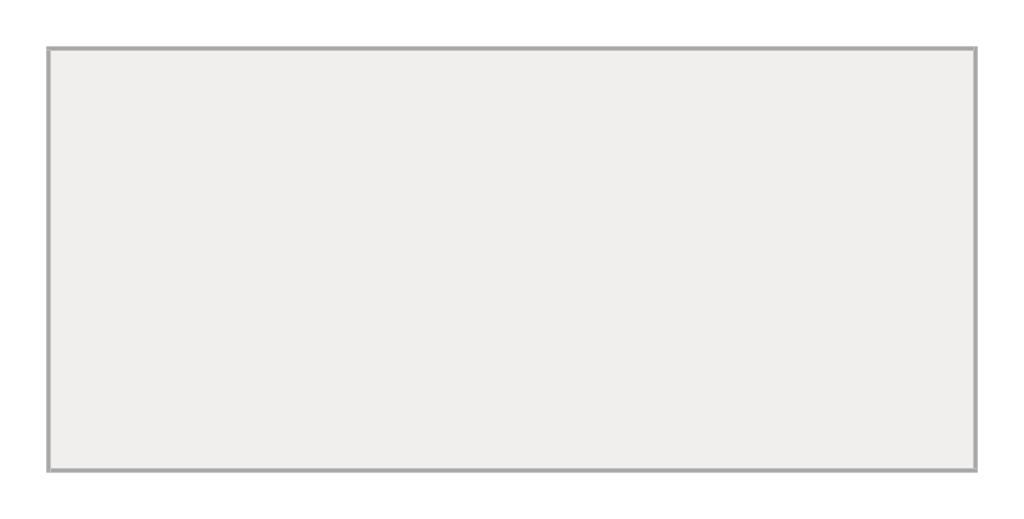
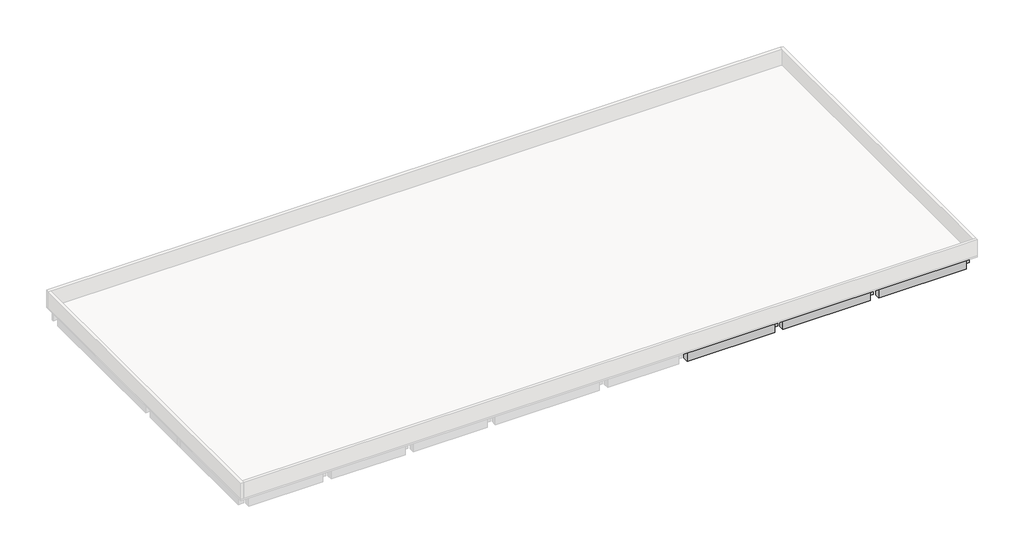
# One storey, part 2 of 2: 30 beams.
"""IFC4 building model written with IfcOpenShell, lengths in millimetres."""

import ifcopenshell
import ifcopenshell.guid

model = None  # the IFC model being written
_history = None  # IfcOwnerHistory: only IFC2X3 demands one
_inside = {}  # id of a spatial element -> (the spatial element, [elements in it])
_under = {}  # id of a project, library or spatial element -> (it, [spatial elements below it])
_declared = {}  # id of a project -> (the project, [libraries it declares])
_typed = {}  # id of a type object -> (the type object, [elements of that type])
_made_of = {}  # id of a material, layer set ... -> (it, [elements and type objects made of it])


def new_model(schema):
    """Start an empty IFC model of exactly this schema.

    Asked for "IFC4X3", IfcOpenShell would pick the latest addendum, in which some entities
    have other attributes; the version numbers below select the first issue.
    IFC2X3 requires an IfcOwnerHistory on every rooted entity: one is made here for all.
    """
    global model, _history
    if schema == "IFC4X3":
        model = ifcopenshell.file(schema_version=(4, 3, 0, 0))
    else:
        model = ifcopenshell.file(schema=schema)
    _inside.clear()
    _under.clear()
    _declared.clear()
    _typed.clear()
    _made_of.clear()
    _history = None
    if model.schema == "IFC2X3":
        org = make("IfcOrganization", Name="unknown")
        user = make(
            "IfcPersonAndOrganization",
            ThePerson=make("IfcPerson", FamilyName="unknown"),
            TheOrganization=org,
        )
        app = make(
            "IfcApplication",
            ApplicationDeveloper=org,
            Version="unknown",
            ApplicationFullName="unknown",
            ApplicationIdentifier="unknown",
        )
        _history = make(
            "IfcOwnerHistory",
            OwningUser=user,
            OwningApplication=app,
            ChangeAction="ADDED",
            CreationDate=0,
        )
    return model


def make(cls, **values):
    """One entity of the class cls with the attributes given. An attribute that is None is left unset."""
    return model.create_entity(
        cls, **{name: value for name, value in values.items() if value is not None}
    )


def rooted(cls, **values):
    """An entity with a GlobalId (a new one), such as an element, a storey or a relation."""
    return make(cls, GlobalId=ifcopenshell.guid.new(), OwnerHistory=_history, **values)


def si_unit(unit_type, name, prefix=None):
    """IfcSIUnit, for example si_unit("LENGTHUNIT", "METRE", prefix="MILLI")."""
    return make("IfcSIUnit", UnitType=unit_type, Prefix=prefix, Name=name)


def assignment(units):
    """IfcUnitAssignment: the units of a project."""
    return None if units is None else make("IfcUnitAssignment", Units=units)


def point(xyz):
    """IfcCartesianPoint."""
    return None if xyz is None else make("IfcCartesianPoint", Coordinates=xyz)


def direction(xyz):
    """IfcDirection."""
    return None if xyz is None else make("IfcDirection", DirectionRatios=xyz)


def frame(location, z_axis=None, x_axis=None):
    """IfcAxis2Placement3D, a coordinate frame: its origin and axes. An axis left out is left unset."""
    return make(
        "IfcAxis2Placement3D",
        Location=point(location),
        Axis=direction(z_axis),
        RefDirection=direction(x_axis),
    )


def origin():
    """The frame at (0, 0, 0) with its axes left unset."""
    return frame((0.0, 0.0, 0.0))


def place(relative_to, where):
    """IfcLocalPlacement: puts the frame where relative to a parent placement (None: the world)."""
    return make(
        "IfcLocalPlacement", PlacementRelTo=relative_to, RelativePlacement=where
    )


def context(
    kind, dimensions, precision=None, world=None, true_north=None, identifier=None
):
    """IfcGeometricRepresentationContext, for example the 3D "Model" context."""
    return make(
        "IfcGeometricRepresentationContext",
        ContextIdentifier=identifier,
        ContextType=kind,
        CoordinateSpaceDimension=dimensions,
        Precision=precision,
        WorldCoordinateSystem=world,
        TrueNorth=true_north,
    )


def project(units=None, contexts=None):
    """IfcProject with its units and contexts."""
    return rooted(
        "IfcProject",
        Name="project",
        RepresentationContexts=contexts,
        UnitsInContext=assignment(units),
    )


def spatial(cls, under=None, at=None, **own):
    """A site, building, storey or space (cls), placed at a placement, below another one or the project."""
    s = rooted(cls, ObjectPlacement=at, **own)
    if under is not None:
        _under.setdefault(under.id(), (under, []))[1].append(s)
    return s


def polyline(points):
    """IfcPolyline through the points."""
    return make("IfcPolyline", Points=[point(p) for p in points])


def outline(outer, holes=None, kind="AREA"):
    """IfcArbitraryClosedProfileDef: a profile drawn as a closed curve; with holes, ...WithVoids."""
    if holes is None:
        return make("IfcArbitraryClosedProfileDef", ProfileType=kind, OuterCurve=outer)
    return make(
        "IfcArbitraryProfileDefWithVoids",
        ProfileType=kind,
        OuterCurve=outer,
        InnerCurves=holes,
    )


def extrude(swept, where, along, depth):
    """IfcExtrudedAreaSolid: the profile swept, set in the frame where, extruded along a direction by depth."""
    return make(
        "IfcExtrudedAreaSolid",
        SweptArea=swept,
        Position=where,
        ExtrudedDirection=direction(along),
        Depth=depth,
    )


def faces_of(points, faces, orient=None, outer=None):
    """IfcFace entities. A face is a list of loops; a loop is a list of indices into points, from 0.

    orient and outer hold one flag for each loop. By default every Orientation is true, the
    first loop of a face is its IfcFaceOuterBound and the others are IfcFaceBound.
    """
    made = []
    for i, loops in enumerate(faces):
        bounds = []
        for j, loop in enumerate(loops):
            is_outer = j == 0 if outer is None else outer[i][j]
            bounds.append(
                make(
                    "IfcFaceOuterBound" if is_outer else "IfcFaceBound",
                    Bound=make("IfcPolyLoop", Polygon=[points[k] for k in loop]),
                    Orientation=True if orient is None else orient[i][j],
                )
            )
        made.append(make("IfcFace", Bounds=bounds))
    return made


def faceted_brep(points, faces, orient=None, outer=None, voids=None):
    """IfcFacetedBrep: a solid bounded by flat faces; with voids (closed shells), ...WithVoids."""
    shared = [point(p) for p in points]
    hull = make("IfcClosedShell", CfsFaces=faces_of(shared, faces, orient, outer))
    if voids is None:
        return make("IfcFacetedBrep", Outer=hull)
    return make(
        "IfcFacetedBrepWithVoids",
        Outer=hull,
        Voids=[
            make(cls, CfsFaces=faces_of(shared, fs, o, b)) for cls, fs, o, b in voids
        ],
    )


def shape(context_of_items, identifier, shape_type, items):
    """IfcShapeRepresentation: the items that make up one representation, for example the "Body"."""
    return make(
        "IfcShapeRepresentation",
        ContextOfItems=context_of_items,
        RepresentationIdentifier=identifier,
        RepresentationType=shape_type,
        Items=items,
    )


def made_of(thing, what):
    """Note that an element or type object is made of a material, layer set ...; save() writes the relation."""
    if what is not None:
        _made_of.setdefault(what.id(), (what, []))[1].append(thing)
    return thing


def element(
    cls,
    number,
    at=None,
    inside=None,
    cuts=None,
    type_object=None,
    material=None,
    context=None,
    identifier="Body",
    shape_type=None,
    held_by="IfcProductDefinitionShape",
    body=None,
    shapes=None,
    **own,
):
    """One element of the class cls, such as IfcWall. Its Tag is "e" and its number.

    at: its placement. inside: the storey or other place that contains it. cuts: it is an
    opening in that element (IfcRelVoidsElement). A single representation is given by context,
    identifier, shape_type and body (its items); several are given by shapes. held_by: the class
    of the entity that holds the representations. save() writes the other relations.
    """
    e = rooted(cls, Tag="e%d" % number, ObjectPlacement=at, **own)
    if body is not None:
        shapes = [shape(context, identifier, shape_type, body)]
    if shapes is not None:
        e.Representation = make(held_by, Representations=shapes)
    if inside is not None:
        _inside.setdefault(inside.id(), (inside, []))[1].append(e)
    if cuts is not None:
        rooted(
            "IfcRelVoidsElement", RelatingBuildingElement=cuts, RelatedOpeningElement=e
        )
    if type_object is not None:
        _typed.setdefault(type_object.id(), (type_object, []))[1].append(e)
    return made_of(e, material)


def aggregate(whole, parts):
    """IfcRelAggregates: a whole, such as a stair, and the parts it consists of."""
    return rooted("IfcRelAggregates", RelatingObject=whole, RelatedObjects=parts)


def save(model, path):
    """Write the relations noted so far, then the file.

    IfcRelAggregates (storeys below a building ...), IfcRelContainedInSpatialStructure (elements
    in a storey), IfcRelDefinesByType, IfcRelAssociatesMaterial and IfcRelDeclares: one each for
    every whole, place, type object, material and project.
    """
    for whole, parts in _under.values():
        aggregate(whole, parts)
    for where, things in _inside.values():
        rooted(
            "IfcRelContainedInSpatialStructure",
            RelatedElements=things,
            RelatingStructure=where,
        )
    for kind, things in _typed.values():
        rooted("IfcRelDefinesByType", RelatedObjects=things, RelatingType=kind)
    for what, things in _made_of.values():
        rooted("IfcRelAssociatesMaterial", RelatedObjects=things, RelatingMaterial=what)
    for by, libraries in _declared.values():
        rooted("IfcRelDeclares", RelatingContext=by, RelatedDefinitions=libraries)
    model.write(path)


model = new_model("IFC4")

# Units and contexts
model_context = context("Model", 3, world=origin())
ifc_project = project(units=[si_unit("LENGTHUNIT", "METRE", prefix="MILLI")], contexts=[model_context])

# Site, building, storey
site = spatial("IfcSite", under=ifc_project)
building = spatial("IfcBuilding", under=site)
storey = spatial("IfcBuildingStorey", under=building, Name="TOC", Elevation=7650.0)

# Beams
placement = place(None, origin())
element("IfcBeam", 1, ObjectType="RC Beam_Rectangular : H_SB_ACB_B400xH900", at=placement, inside=storey, context=model_context, shape_type="Brep", body=[
    faceted_brep([(39124.7, 12116.5208589, 6750.0), (39124.7, 12116.5208589, 7549.0), (38724.7, 12116.5208589, 7549.0), (32124.7, 12116.5208589, 7549.0), (32124.7, 12116.5208589, 6750.0), (38724.7, 12116.5208589, 6750.0), (39124.7, 12516.5208589, 6750.0), (32124.7, 12516.5208589, 6750.0), (38724.7, 12516.5208589, 6750.0), (39124.7, 12516.5208589, 7549.0), (32124.7, 12516.5208589, 7549.0), (38724.7, 12516.5208589, 7549.0)], [[[0, 1, 2, 3, 4, 5]], [[6, 0, 5, 4, 7, 8]], [[9, 6, 8, 7, 10, 11]], [[1, 9, 11, 10, 3, 2]], [[0, 6, 9, 1]], [[4, 3, 10, 7]]]),
])
element("IfcBeam", 2, ObjectType="RC Beam_Rectangular : H_SB_ACB_B400xH900", at=placement, inside=storey, context=model_context, shape_type="Brep", body=[
    faceted_brep([(46124.7, 12116.5208589, 6750.0), (46124.7, 12116.5208589, 7549.0), (45724.7, 12116.5208589, 7549.0), (39124.7, 12116.5208589, 7549.0), (39124.7, 12116.5208589, 6750.0), (45724.7, 12116.5208589, 6750.0), (46124.7, 12516.5208589, 6750.0), (39124.7, 12516.5208589, 6750.0), (45724.7, 12516.5208589, 6750.0), (46124.7, 12516.5208589, 7549.0), (39124.7, 12516.5208589, 7549.0), (45724.7, 12516.5208589, 7549.0)], [[[0, 1, 2, 3, 4, 5]], [[6, 0, 5, 4, 7, 8]], [[9, 6, 8, 7, 10, 11]], [[1, 9, 11, 10, 3, 2]], [[0, 6, 9, 1]], [[4, 3, 10, 7]]]),
])
element("IfcBeam", 3, ObjectType="RC Beam_Rectangular : H_SB_ACB_B400xH900", at=placement, inside=storey, context=model_context, shape_type="Brep", body=[
    faceted_brep([(53124.7, 12116.5208589, 6750.0), (53124.7, 12116.5208589, 7549.0), (52724.7, 12116.5208589, 7549.0), (46124.7, 12116.5208589, 7549.0), (46124.7, 12116.5208589, 6750.0), (52724.7, 12116.5208589, 6750.0), (53124.7, 12516.5208589, 6750.0), (46124.7, 12516.5208589, 6750.0), (52724.7, 12516.5208589, 6750.0), (53124.7, 12516.5208589, 7549.0), (46124.7, 12516.5208589, 7549.0), (52724.7, 12516.5208589, 7549.0)], [[[0, 1, 2, 3, 4, 5]], [[6, 0, 5, 4, 7, 8]], [[9, 6, 8, 7, 10, 11]], [[1, 9, 11, 10, 3, 2]], [[0, 6, 9, 1]], [[4, 3, 10, 7]]]),
])
element("IfcBeam", 4, ObjectType="RC Beam_Rectangular : H_SB_ACB_B400xH900", at=placement, inside=storey, context=model_context, shape_type="SweptSolid", body=[
    extrude(outline(polyline([(7500.0, 224.7), (6750.0, 224.7), (6750.0, 5624.7), (7500.0, 5624.7), (7500.0, 5724.7), (7549.0, 5724.7), (7549.0, 124.7), (7500.0, 124.7), (7500.0, 224.7)])), frame((0.0, 23816.5208589, 0.0), z_axis=(0.0, 1.0, 0.0), x_axis=(0.0, 0.0, 1.0)), (0.0, 0.0, 1.0), 400.0),
])
element("IfcBeam", 5, ObjectType="RC Beam_Rectangular : H_SB_ACB_B400xH900", at=placement, inside=storey, context=model_context, shape_type="SweptSolid", body=[
    extrude(outline(polyline([(7500.0, 6224.7), (6750.0, 6224.7), (6750.0, 11624.7), (7500.0, 11624.7), (7500.0, 11724.7), (7549.0, 11724.7), (7549.0, 6124.7), (7500.0, 6124.7), (7500.0, 6224.7)])), frame((0.0, 23816.5208589, 0.0), z_axis=(0.0, 1.0, 0.0), x_axis=(0.0, 0.0, 1.0)), (0.0, 0.0, 1.0), 400.0),
])
element("IfcBeam", 6, ObjectType="RC Beam_Rectangular : H_SB_ACB_B400xH900", at=placement, inside=storey, context=model_context, shape_type="SweptSolid", body=[
    extrude(outline(polyline([(7500.0, 12224.7), (6750.0, 12224.7), (6750.0, 17624.7), (7500.0, 17624.7), (7500.0, 17724.7), (7549.0, 17724.7), (7549.0, 12124.7), (7500.0, 12124.7), (7500.0, 12224.7)])), frame((0.0, 23816.5208589, 0.0), z_axis=(0.0, 1.0, 0.0), x_axis=(0.0, 0.0, 1.0)), (0.0, 0.0, 1.0), 400.0),
])
element("IfcBeam", 7, ObjectType="RC Beam_Rectangular : H_SB_ACB_B400xH900", at=placement, inside=storey, context=model_context, shape_type="SweptSolid", body=[
    extrude(outline(polyline([(7500.0, 18224.7), (6750.0, 18224.7), (6750.0, 25824.7), (7500.0, 25824.7), (7500.0, 25924.7), (7549.0, 25924.7), (7549.0, 18124.7), (7500.0, 18124.7), (7500.0, 18224.7)])), frame((0.0, 23816.5208589, 0.0), z_axis=(0.0, 1.0, 0.0), x_axis=(0.0, 0.0, 1.0)), (0.0, 0.0, 1.0), 400.0),
])
element("IfcBeam", 8, ObjectType="RC Beam_Rectangular : H_SB_ACB_B400xH900", at=placement, inside=storey, context=model_context, shape_type="SweptSolid", body=[
    extrude(outline(polyline([(7500.0, 26424.7), (6750.0, 26424.7), (6750.0, 31624.7), (7500.0, 31624.7), (7500.0, 31724.7), (7549.0, 31724.7), (7549.0, 26324.7), (7500.0, 26324.7), (7500.0, 26424.7)])), frame((0.0, 23816.5208589, 0.0), z_axis=(0.0, 1.0, 0.0), x_axis=(0.0, 0.0, 1.0)), (0.0, 0.0, 1.0), 400.0),
])
element("IfcBeam", 9, ObjectType="RC Beam_Rectangular : H_SB_ACB_B400xH900", at=placement, inside=storey, context=model_context, shape_type="SweptSolid", body=[
    extrude(outline(polyline([(7500.0, 32224.7), (6750.0, 32224.7), (6750.0, 38624.7), (7500.0, 38624.7), (7500.0, 38724.7), (7549.0, 38724.7), (7549.0, 32124.7), (7500.0, 32124.7), (7500.0, 32224.7)])), frame((0.0, 23816.5208589, 0.0), z_axis=(0.0, 1.0, 0.0), x_axis=(0.0, 0.0, 1.0)), (0.0, 0.0, 1.0), 400.0),
])
element("IfcBeam", 10, ObjectType="RC Beam_Rectangular : H_SB_ACB_B400xH900", at=placement, inside=storey, context=model_context, shape_type="SweptSolid", body=[
    extrude(outline(polyline([(7500.0, 39224.7), (6750.0, 39224.7), (6750.0, 45624.7), (7500.0, 45624.7), (7500.0, 45724.7), (7549.0, 45724.7), (7549.0, 39124.7), (7500.0, 39124.7), (7500.0, 39224.7)])), frame((0.0, 23816.5208589, 0.0), z_axis=(0.0, 1.0, 0.0), x_axis=(0.0, 0.0, 1.0)), (0.0, 0.0, 1.0), 400.0),
])
element("IfcBeam", 11, ObjectType="RC Beam_Rectangular : H_SB_ACB_B400xH900", at=placement, inside=storey, context=model_context, shape_type="SweptSolid", body=[
    extrude(outline(polyline([(7500.0, 46224.7), (6750.0, 46224.7), (6750.0, 52624.7), (7500.0, 52624.7), (7500.0, 52724.7), (7549.0, 52724.7), (7549.0, 46124.7), (7500.0, 46124.7), (7500.0, 46224.7)])), frame((0.0, 23816.5208589, 0.0), z_axis=(0.0, 1.0, 0.0), x_axis=(0.0, 0.0, 1.0)), (0.0, 0.0, 1.0), 400.0),
])
element("IfcBeam", 12, ObjectType="RC Beam_Rectangular : H_SB_ACB_B400xH900", at=placement, inside=storey, context=model_context, shape_type="Brep", body=[
    faceted_brep([(32224.7, 8216.5208589, 7500.0), (32224.7, 8216.5208589, 6750.0), (38624.7, 8216.5208589, 6750.0), (38624.7, 8216.5208589, 7500.0), (38724.7, 8216.5208589, 7500.0), (39124.7, 8216.5208589, 7500.0), (39124.7, 8216.5208589, 7549.0), (38724.7, 8216.5208589, 7549.0), (32124.7, 8216.5208589, 7549.0), (32124.7, 8216.5208589, 7500.0), (32224.7, 8616.5208589, 6750.0), (38624.7, 8616.5208589, 6750.0), (32224.7, 8616.5208589, 7500.0), (32124.7, 8616.5208589, 7500.0), (32124.7, 8616.5208589, 7549.0), (38724.7, 8616.5208589, 7549.0), (39124.7, 8616.5208589, 7549.0), (39124.7, 8616.5208589, 7500.0), (38724.7, 8616.5208589, 7500.0), (38624.7, 8616.5208589, 7500.0)], [[[0, 1, 2, 3, 4, 5, 6, 7, 8, 9]], [[1, 10, 11, 2]], [[10, 12, 13, 14, 15, 16, 17, 18, 19, 11]], [[1, 0, 12, 10]], [[0, 9, 13, 12]], [[19, 3, 2, 11]], [[3, 19, 18, 17, 5, 4]], [[8, 7, 6, 16, 15, 14]], [[16, 6, 5, 17]], [[8, 14, 13, 9]]]),
])
element("IfcBeam", 13, ObjectType="RC Beam_Rectangular : H_SB_ACB_B400xH900", at=placement, inside=storey, context=model_context, shape_type="Brep", body=[
    faceted_brep([(39224.7, 8216.5208589, 7500.0), (39224.7, 8216.5208589, 6750.0), (45624.7, 8216.5208589, 6750.0), (45624.7, 8216.5208589, 7500.0), (45724.7, 8216.5208589, 7500.0), (46124.7, 8216.5208589, 7500.0), (46124.7, 8216.5208589, 7549.0), (45724.7, 8216.5208589, 7549.0), (39124.7, 8216.5208589, 7549.0), (39124.7, 8216.5208589, 7500.0), (39224.7, 8616.5208589, 6750.0), (45624.7, 8616.5208589, 6750.0), (39224.7, 8616.5208589, 7500.0), (39124.7, 8616.5208589, 7500.0), (39124.7, 8616.5208589, 7549.0), (45724.7, 8616.5208589, 7549.0), (46124.7, 8616.5208589, 7549.0), (46124.7, 8616.5208589, 7500.0), (45724.7, 8616.5208589, 7500.0), (45624.7, 8616.5208589, 7500.0)], [[[0, 1, 2, 3, 4, 5, 6, 7, 8, 9]], [[1, 10, 11, 2]], [[10, 12, 13, 14, 15, 16, 17, 18, 19, 11]], [[1, 0, 12, 10]], [[0, 9, 13, 12]], [[19, 3, 2, 11]], [[3, 19, 18, 17, 5, 4]], [[8, 7, 6, 16, 15, 14]], [[16, 6, 5, 17]], [[8, 14, 13, 9]]]),
])
element("IfcBeam", 14, ObjectType="RC Beam_Rectangular : H_SB_ACB_B400xH900", at=placement, inside=storey, context=model_context, shape_type="Brep", body=[
    faceted_brep([(46224.7, 8216.5208589, 7500.0), (46224.7, 8216.5208589, 6750.0), (52624.7, 8216.5208589, 6750.0), (52624.7, 8216.5208589, 7500.0), (52724.7, 8216.5208589, 7500.0), (53124.7, 8216.5208589, 7500.0), (53124.7, 8216.5208589, 7549.0), (52724.7, 8216.5208589, 7549.0), (46124.7, 8216.5208589, 7549.0), (46124.7, 8216.5208589, 7500.0), (46224.7, 8616.5208589, 6750.0), (52624.7, 8616.5208589, 6750.0), (46224.7, 8616.5208589, 7500.0), (46124.7, 8616.5208589, 7500.0), (46124.7, 8616.5208589, 7549.0), (52724.7, 8616.5208589, 7549.0), (53124.7, 8616.5208589, 7549.0), (53124.7, 8616.5208589, 7500.0), (52724.7, 8616.5208589, 7500.0), (52624.7, 8616.5208589, 7500.0)], [[[0, 1, 2, 3, 4, 5, 6, 7, 8, 9]], [[1, 10, 11, 2]], [[10, 12, 13, 14, 15, 16, 17, 18, 19, 11]], [[1, 0, 12, 10]], [[0, 9, 13, 12]], [[19, 3, 2, 11]], [[3, 19, 18, 17, 5, 4]], [[8, 7, 6, 16, 15, 14]], [[16, 6, 5, 17]], [[8, 14, 13, 9]]]),
])
element("IfcBeam", 15, ObjectType="RC Beam_Rectangular : H_SB_ACB_B400xH900", at=placement, inside=storey, context=model_context, shape_type="Brep", body=[
    faceted_brep([(32224.7, 416.5208589, 7500.0), (32224.7, 416.5208589, 6750.0), (38624.7, 416.5208589, 6750.0), (38624.7, 416.5208589, 7500.0), (39124.7, 416.5208589, 7500.0), (39124.7, 416.5208589, 7549.0), (32124.7, 416.5208589, 7549.0), (32124.7, 416.5208589, 7500.0), (32224.7, 816.5208589, 6750.0), (38624.7, 816.5208589, 6750.0), (32224.7, 816.5208589, 7500.0), (32124.7, 816.5208589, 7500.0), (32124.7, 816.5208589, 7549.0), (38724.7, 816.5208589, 7549.0), (39124.7, 816.5208589, 7549.0), (39124.7, 816.5208589, 7500.0), (38724.7, 816.5208589, 7500.0), (38624.7, 816.5208589, 7500.0)], [[[0, 1, 2, 3, 4, 5, 6, 7]], [[1, 8, 9, 2]], [[8, 10, 11, 12, 13, 14, 15, 16, 17, 9]], [[8, 1, 0, 10]], [[11, 10, 0, 7]], [[17, 3, 2, 9]], [[3, 17, 16, 15, 4]], [[6, 5, 14, 13, 12]], [[14, 5, 4, 15]], [[6, 12, 11, 7]]]),
])
element("IfcBeam", 16, ObjectType="RC Beam_Rectangular : H_SB_ACB_B400xH900", at=placement, inside=storey, context=model_context, shape_type="Brep", body=[
    faceted_brep([(39224.7, 416.5208589, 7500.0), (39224.7, 416.5208589, 6750.0), (45624.7, 416.5208589, 6750.0), (45624.7, 416.5208589, 7500.0), (46124.7, 416.5208589, 7500.0), (46124.7, 416.5208589, 7549.0), (39124.7, 416.5208589, 7549.0), (39124.7, 416.5208589, 7500.0), (39224.7, 816.5208589, 6750.0), (45624.7, 816.5208589, 6750.0), (39224.7, 816.5208589, 7500.0), (39124.7, 816.5208589, 7500.0), (39124.7, 816.5208589, 7549.0), (45724.7, 816.5208589, 7549.0), (46124.7, 816.5208589, 7549.0), (46124.7, 816.5208589, 7500.0), (45724.7, 816.5208589, 7500.0), (45624.7, 816.5208589, 7500.0)], [[[0, 1, 2, 3, 4, 5, 6, 7]], [[1, 8, 9, 2]], [[8, 10, 11, 12, 13, 14, 15, 16, 17, 9]], [[8, 1, 0, 10]], [[11, 10, 0, 7]], [[17, 3, 2, 9]], [[3, 17, 16, 15, 4]], [[6, 5, 14, 13, 12]], [[14, 5, 4, 15]], [[6, 12, 11, 7]]]),
])
element("IfcBeam", 17, ObjectType="RC Beam_Rectangular : H_SB_ACB_B400xH900", at=placement, inside=storey, context=model_context, shape_type="Brep", body=[
    faceted_brep([(46224.7, 416.5208589, 7500.0), (46224.7, 416.5208589, 6750.0), (52624.7, 416.5208589, 6750.0), (52624.7, 416.5208589, 7500.0), (53124.7, 416.5208589, 7500.0), (53124.7, 416.5208589, 7549.0), (46124.7, 416.5208589, 7549.0), (46124.7, 416.5208589, 7500.0), (46224.7, 816.5208589, 6750.0), (52624.7, 816.5208589, 6750.0), (46224.7, 816.5208589, 7500.0), (46124.7, 816.5208589, 7500.0), (46124.7, 816.5208589, 7549.0), (52724.7, 816.5208589, 7549.0), (53124.7, 816.5208589, 7549.0), (53124.7, 816.5208589, 7500.0), (52724.7, 816.5208589, 7500.0), (52624.7, 816.5208589, 7500.0)], [[[0, 1, 2, 3, 4, 5, 6, 7]], [[1, 8, 9, 2]], [[8, 10, 11, 12, 13, 14, 15, 16, 17, 9]], [[8, 1, 0, 10]], [[11, 10, 0, 7]], [[17, 3, 2, 9]], [[3, 17, 16, 15, 4]], [[6, 5, 14, 13, 12]], [[14, 5, 4, 15]], [[6, 12, 11, 7]]]),
])
element("IfcBeam", 18, ObjectType="RC Beam_Rectangular : H_SB_ACB_B400xH900", at=placement, inside=storey, context=model_context, shape_type="Brep", body=[
    faceted_brep([(12124.7, 24429.2208589, 6750.0), (11724.7, 24429.2208589, 6750.0), (11724.7, 24429.2208589, 7549.0), (12124.7, 24429.2208589, 7549.0), (12124.7, 12616.5208589, 7500.0), (12124.7, 12616.5208589, 6750.0), (12124.7, 23716.5208589, 6750.0), (12124.7, 23716.5208589, 7500.0), (12124.7, 23816.5208589, 7500.0), (12124.7, 24216.5208589, 7500.0), (12124.7, 24316.5208589, 7500.0), (12124.7, 24316.5208589, 6750.0), (12124.7, 24216.5208589, 7549.0), (12124.7, 23816.5208589, 7549.0), (12124.7, 12516.5208589, 7549.0), (12124.7, 12516.5208589, 7500.0), (11724.7, 24316.5208589, 6750.0), (11724.7, 24316.5208589, 7500.0), (11724.7, 24216.5208589, 7500.0), (11724.7, 23816.5208589, 7500.0), (11724.7, 23716.5208589, 7500.0), (11724.7, 23716.5208589, 6750.0), (11724.7, 12616.5208589, 6750.0), (11724.7, 12616.5208589, 7500.0), (11724.7, 12516.5208589, 7500.0), (11724.7, 12516.5208589, 7549.0), (11724.7, 23816.5208589, 7549.0), (11724.7, 24216.5208589, 7549.0)], [[[0, 1, 2, 3]], [[4, 5, 6, 7, 8, 9, 10, 11, 0, 3, 12, 13, 14, 15]], [[1, 0, 11, 16]], [[2, 1, 16, 17, 18, 19, 20, 21, 22, 23, 24, 25, 26, 27]], [[24, 15, 14, 25]], [[5, 4, 23, 22]], [[4, 15, 24, 23]], [[20, 7, 6, 21]], [[7, 20, 19, 18, 17, 10, 9, 8]], [[3, 2, 27, 26, 25, 14, 13, 12]], [[10, 17, 16, 11]], [[5, 22, 21, 6]]]),
])
element("IfcBeam", 19, ObjectType="RC Beam_Rectangular : H_SB_ACB_B400xH900", at=placement, inside=storey, context=model_context, shape_type="Brep", body=[
    faceted_brep([(18124.7, 24429.2208589, 6750.0), (17724.7, 24429.2208589, 6750.0), (17724.7, 24429.2208589, 7549.0), (18124.7, 24429.2208589, 7549.0), (18124.7, 12616.5208589, 7500.0), (18124.7, 12616.5208589, 6750.0), (18124.7, 23716.5208589, 6750.0), (18124.7, 23716.5208589, 7500.0), (18124.7, 23816.5208589, 7500.0), (18124.7, 24216.5208589, 7500.0), (18124.7, 24316.5208589, 7500.0), (18124.7, 24316.5208589, 6750.0), (18124.7, 24216.5208589, 7549.0), (18124.7, 23816.5208589, 7549.0), (18124.7, 12516.5208589, 7549.0), (18124.7, 12516.5208589, 7500.0), (17724.7, 24316.5208589, 6750.0), (17724.7, 24316.5208589, 7500.0), (17724.7, 24216.5208589, 7500.0), (17724.7, 23816.5208589, 7500.0), (17724.7, 23716.5208589, 7500.0), (17724.7, 23716.5208589, 6750.0), (17724.7, 12616.5208589, 6750.0), (17724.7, 12616.5208589, 7500.0), (17724.7, 12516.5208589, 7500.0), (17724.7, 12516.5208589, 7549.0), (17724.7, 23816.5208589, 7549.0), (17724.7, 24216.5208589, 7549.0)], [[[0, 1, 2, 3]], [[4, 5, 6, 7, 8, 9, 10, 11, 0, 3, 12, 13, 14, 15]], [[1, 0, 11, 16]], [[2, 1, 16, 17, 18, 19, 20, 21, 22, 23, 24, 25, 26, 27]], [[24, 15, 14, 25]], [[5, 4, 23, 22]], [[4, 15, 24, 23]], [[20, 7, 6, 21]], [[7, 20, 19, 18, 17, 10, 9, 8]], [[3, 2, 27, 26, 25, 14, 13, 12]], [[10, 17, 16, 11]], [[5, 22, 21, 6]]]),
])
element("IfcBeam", 20, ObjectType="RC Beam_Rectangular : H_SB_ACB_B400xH900", at=placement, inside=storey, context=model_context, shape_type="Brep", body=[
    faceted_brep([(26324.7, 24429.2208589, 6750.0), (25924.7, 24429.2208589, 6750.0), (25924.7, 24429.2208589, 7549.0), (26324.7, 24429.2208589, 7549.0), (26324.7, 24216.5208589, 7549.0), (26324.7, 23816.5208589, 7549.0), (26324.7, 12516.5208589, 7549.0), (26324.7, 12516.5208589, 6750.0), (26324.7, 23716.5208589, 6750.0), (26324.7, 23716.5208589, 7500.0), (26324.7, 23816.5208589, 7500.0), (26324.7, 24216.5208589, 7500.0), (26324.7, 24316.5208589, 7500.0), (26324.7, 24316.5208589, 6750.0), (25924.7, 24316.5208589, 6750.0), (25924.7, 12516.5208589, 6750.0), (25924.7, 12516.5208589, 7549.0), (25924.7, 23816.5208589, 7549.0), (25924.7, 24216.5208589, 7549.0), (25924.7, 24316.5208589, 7500.0), (25924.7, 24216.5208589, 7500.0), (25924.7, 23816.5208589, 7500.0), (25924.7, 23716.5208589, 7500.0), (25924.7, 23716.5208589, 6750.0)], [[[0, 1, 2, 3]], [[0, 3, 4, 5, 6, 7, 8, 9, 10, 11, 12, 13]], [[1, 0, 13, 14]], [[15, 16, 17, 18, 2, 1, 14, 19, 20, 21, 22, 23]], [[15, 7, 6, 16]], [[22, 9, 8, 23]], [[9, 22, 21, 20, 19, 12, 11, 10]], [[3, 2, 18, 17, 16, 6, 5, 4]], [[12, 19, 14, 13]], [[7, 15, 23, 8]]]),
])
element("IfcBeam", 21, ObjectType="RC Beam_Rectangular : H_SB_ACB_B400xH900", at=placement, inside=storey, context=model_context, shape_type="Brep", body=[
    faceted_brep([(32124.7, 24429.2208589, 6750.0), (31724.7, 24429.2208589, 6750.0), (31724.7, 24429.2208589, 7549.0), (32124.7, 24429.2208589, 7549.0), (32124.7, 24216.5208589, 7549.0), (32124.7, 23816.5208589, 7549.0), (32124.7, 12516.5208589, 7549.0), (32124.7, 12516.5208589, 6750.0), (32124.7, 23716.5208589, 6750.0), (32124.7, 23716.5208589, 7500.0), (32124.7, 23816.5208589, 7500.0), (32124.7, 24216.5208589, 7500.0), (32124.7, 24316.5208589, 7500.0), (32124.7, 24316.5208589, 6750.0), (31724.7, 24316.5208589, 6750.0), (31724.7, 12516.5208589, 6750.0), (31724.7, 12516.5208589, 7549.0), (31724.7, 23816.5208589, 7549.0), (31724.7, 24216.5208589, 7549.0), (31724.7, 24316.5208589, 7500.0), (31724.7, 24216.5208589, 7500.0), (31724.7, 23816.5208589, 7500.0), (31724.7, 23716.5208589, 7500.0), (31724.7, 23716.5208589, 6750.0)], [[[0, 1, 2, 3]], [[0, 3, 4, 5, 6, 7, 8, 9, 10, 11, 12, 13]], [[1, 0, 13, 14]], [[15, 16, 17, 18, 2, 1, 14, 19, 20, 21, 22, 23]], [[15, 7, 6, 16]], [[22, 9, 8, 23]], [[9, 22, 21, 20, 19, 12, 11, 10]], [[3, 2, 18, 17, 16, 6, 5, 4]], [[12, 19, 14, 13]], [[7, 15, 23, 8]]]),
])
element("IfcBeam", 22, ObjectType="RC Beam_Rectangular : H_SB_ACB_B400xH900", at=placement, inside=storey, context=model_context, shape_type="SweptSolid", body=[
    extrude(outline(polyline([(8116.5208589, 7500.0), (8116.5208589, 6750.0), (916.5208589, 6750.0), (916.5208589, 7500.0), (816.5208589, 7500.0), (816.5208589, 7549.0), (8216.5208589, 7549.0), (8216.5208589, 7500.0), (8116.5208589, 7500.0)])), frame((38724.7, 0.0, 0.0), z_axis=(1.0, 0.0, 0.0), x_axis=(0.0, 1.0, 0.0)), (0.0, 0.0, 1.0), 400.0),
])
element("IfcBeam", 23, ObjectType="RC Beam_Rectangular : H_SB_ACB_B400xH900", at=placement, inside=storey, context=model_context, shape_type="SweptSolid", body=[
    extrude(outline(polyline([(12116.5208589, 7549.0), (12116.5208589, 6750.0), (8716.5208589, 6750.0), (8716.5208589, 7500.0), (8616.5208589, 7500.0), (8616.5208589, 7549.0), (12116.5208589, 7549.0)])), frame((38724.7, 0.0, 0.0), z_axis=(1.0, 0.0, 0.0), x_axis=(0.0, 1.0, 0.0)), (0.0, 0.0, 1.0), 400.0),
])
element("IfcBeam", 24, ObjectType="RC Beam_Rectangular : H_SB_ACB_B400xH900", at=placement, inside=storey, context=model_context, shape_type="Brep", body=[
    faceted_brep([(39124.7, 24429.2208589, 6750.0), (38724.7, 24429.2208589, 6750.0), (38724.7, 24429.2208589, 7549.0), (39124.7, 24429.2208589, 7549.0), (39124.7, 24216.5208589, 7549.0), (39124.7, 23816.5208589, 7549.0), (39124.7, 12516.5208589, 7549.0), (39124.7, 12516.5208589, 6750.0), (39124.7, 23716.5208589, 6750.0), (39124.7, 23716.5208589, 7500.0), (39124.7, 23816.5208589, 7500.0), (39124.7, 24216.5208589, 7500.0), (39124.7, 24316.5208589, 7500.0), (39124.7, 24316.5208589, 6750.0), (38724.7, 24316.5208589, 6750.0), (38724.7, 12516.5208589, 6750.0), (38724.7, 12516.5208589, 7549.0), (38724.7, 23816.5208589, 7549.0), (38724.7, 24216.5208589, 7549.0), (38724.7, 24316.5208589, 7500.0), (38724.7, 24216.5208589, 7500.0), (38724.7, 23816.5208589, 7500.0), (38724.7, 23716.5208589, 7500.0), (38724.7, 23716.5208589, 6750.0)], [[[0, 1, 2, 3]], [[0, 3, 4, 5, 6, 7, 8, 9, 10, 11, 12, 13]], [[1, 0, 13, 14]], [[15, 16, 17, 18, 2, 1, 14, 19, 20, 21, 22, 23]], [[15, 7, 6, 16]], [[22, 9, 8, 23]], [[9, 22, 21, 20, 19, 12, 11, 10]], [[3, 2, 18, 17, 16, 6, 5, 4]], [[12, 19, 14, 13]], [[7, 15, 23, 8]]]),
])
element("IfcBeam", 25, ObjectType="RC Beam_Rectangular : H_SB_ACB_B400xH900", at=placement, inside=storey, context=model_context, shape_type="SweptSolid", body=[
    extrude(outline(polyline([(8116.5208589, 7500.0), (8116.5208589, 6750.0), (916.5208589, 6750.0), (916.5208589, 7500.0), (816.5208589, 7500.0), (816.5208589, 7549.0), (8216.5208589, 7549.0), (8216.5208589, 7500.0), (8116.5208589, 7500.0)])), frame((45724.7, 0.0, 0.0), z_axis=(1.0, 0.0, 0.0), x_axis=(0.0, 1.0, 0.0)), (0.0, 0.0, 1.0), 400.0),
])
element("IfcBeam", 26, ObjectType="RC Beam_Rectangular : H_SB_ACB_B400xH900", at=placement, inside=storey, context=model_context, shape_type="SweptSolid", body=[
    extrude(outline(polyline([(12116.5208589, 7549.0), (12116.5208589, 6750.0), (8716.5208589, 6750.0), (8716.5208589, 7500.0), (8616.5208589, 7500.0), (8616.5208589, 7549.0), (12116.5208589, 7549.0)])), frame((45724.7, 0.0, 0.0), z_axis=(1.0, 0.0, 0.0), x_axis=(0.0, 1.0, 0.0)), (0.0, 0.0, 1.0), 400.0),
])
element("IfcBeam", 27, ObjectType="RC Beam_Rectangular : H_SB_ACB_B400xH900", at=placement, inside=storey, context=model_context, shape_type="Brep", body=[
    faceted_brep([(46124.7, 24429.2208589, 6750.0), (45724.7, 24429.2208589, 6750.0), (45724.7, 24429.2208589, 7549.0), (46124.7, 24429.2208589, 7549.0), (46124.7, 24216.5208589, 7549.0), (46124.7, 23816.5208589, 7549.0), (46124.7, 12516.5208589, 7549.0), (46124.7, 12516.5208589, 6750.0), (46124.7, 23716.5208589, 6750.0), (46124.7, 23716.5208589, 7500.0), (46124.7, 23816.5208589, 7500.0), (46124.7, 24216.5208589, 7500.0), (46124.7, 24316.5208589, 7500.0), (46124.7, 24316.5208589, 6750.0), (45724.7, 24316.5208589, 6750.0), (45724.7, 12516.5208589, 6750.0), (45724.7, 12516.5208589, 7549.0), (45724.7, 23816.5208589, 7549.0), (45724.7, 24216.5208589, 7549.0), (45724.7, 24316.5208589, 7500.0), (45724.7, 24216.5208589, 7500.0), (45724.7, 23816.5208589, 7500.0), (45724.7, 23716.5208589, 7500.0), (45724.7, 23716.5208589, 6750.0)], [[[0, 1, 2, 3]], [[0, 3, 4, 5, 6, 7, 8, 9, 10, 11, 12, 13]], [[1, 0, 13, 14]], [[15, 16, 17, 18, 2, 1, 14, 19, 20, 21, 22, 23]], [[15, 7, 6, 16]], [[22, 9, 8, 23]], [[9, 22, 21, 20, 19, 12, 11, 10]], [[3, 2, 18, 17, 16, 6, 5, 4]], [[12, 19, 14, 13]], [[7, 15, 23, 8]]]),
])
element("IfcBeam", 28, ObjectType="RC Beam_Rectangular : H_SB_ACB_B400xH900", at=placement, inside=storey, context=model_context, shape_type="SweptSolid", body=[
    extrude(outline(polyline([(8116.5208589, 7500.0), (8116.5208589, 6750.0), (916.5208589, 6750.0), (916.5208589, 7500.0), (816.5208589, 7500.0), (816.5208589, 7549.0), (8216.5208589, 7549.0), (8216.5208589, 7500.0), (8116.5208589, 7500.0)])), frame((52724.7, 0.0, 0.0), z_axis=(1.0, 0.0, 0.0), x_axis=(0.0, 1.0, 0.0)), (0.0, 0.0, 1.0), 400.0),
])
element("IfcBeam", 29, ObjectType="RC Beam_Rectangular : H_SB_ACB_B400xH900", at=placement, inside=storey, context=model_context, shape_type="SweptSolid", body=[
    extrude(outline(polyline([(12116.5208589, 7549.0), (12116.5208589, 6750.0), (8716.5208589, 6750.0), (8716.5208589, 7500.0), (8616.5208589, 7500.0), (8616.5208589, 7549.0), (12116.5208589, 7549.0)])), frame((52724.7, 0.0, 0.0), z_axis=(1.0, 0.0, 0.0), x_axis=(0.0, 1.0, 0.0)), (0.0, 0.0, 1.0), 400.0),
])
element("IfcBeam", 30, ObjectType="RC Beam_Rectangular : H_SB_ACB_B400xH900", at=placement, inside=storey, context=model_context, shape_type="Brep", body=[
    faceted_brep([(53124.7, 24429.2208589, 6750.0), (52724.7, 24429.2208589, 6750.0), (52724.7, 24429.2208589, 7549.0), (53124.7, 24429.2208589, 7549.0), (53124.7, 23716.5208589, 6750.0), (53124.7, 23716.5208589, 7500.0), (53124.7, 24316.5208589, 7500.0), (53124.7, 24316.5208589, 6750.0), (53124.7, 12516.5208589, 7549.0), (53124.7, 12516.5208589, 6750.0), (52724.7, 24316.5208589, 6750.0), (52724.7, 24316.5208589, 7500.0), (52724.7, 24216.5208589, 7500.0), (52724.7, 23816.5208589, 7500.0), (52724.7, 23716.5208589, 7500.0), (52724.7, 23716.5208589, 6750.0), (52724.7, 12516.5208589, 6750.0), (52724.7, 12516.5208589, 7549.0), (52724.7, 23816.5208589, 7549.0), (52724.7, 24216.5208589, 7549.0)], [[[0, 1, 2, 3]], [[4, 5, 6, 7, 0, 3, 8, 9]], [[1, 0, 7, 10]], [[11, 12, 13, 14, 15, 16, 17, 18, 19, 2, 1, 10]], [[4, 15, 14, 5]], [[14, 13, 12, 11, 6, 5]], [[9, 8, 17, 16]], [[3, 2, 19, 18, 17, 8]], [[6, 11, 10, 7]], [[15, 4, 9, 16]]]),
])

save(model, "model.ifc")

# Revit data of these elements
# Type "RC Beam_Rectangular : H_SB_ACB_B400xH900"
#   중앙부 하부근 = ""
#   중앙부 상부근 = ""
#   중앙부 보조근 = ""
#   중앙부 늑근 = ""
#   외단부 하부근 = ""
#   외단부 상부근 = ""
#   외단부 보조근 = ""
#   외단부 늑근 = ""
#   부호 = "TG3"
#   내단부 하부근 = ""
#   내단부 상부근 = ""
#   내단부 보조근 = ""
#   내단부 늑근 = ""
#   ALL 하부근 = "3-D20"
#   ALL 상부근 = "3-D20"
#   ALL 보조근 = ""
#   ALL 늑근 = "2-D10 @120"
#   Width = 400.000 mm
#   Height = 900.000 mm
#   Length [instance default] = 1524.000 mm
#   b = 400.000 mm
#   h = 900.000 mm
#   hec_material3 [instance default] = none
#   hec_material2 [instance default] = none
#   hec_material1 [instance default] = none
#   Structural Material [instance default] = none
#   Assembly Code = ""
# Elements 1, 2, 3, 4, 5, 6, 7, 8, 9, 10, 11, 12, 13, 14, 15, 16, 17, 18, 19, 20, 21, 22, 23, 24, 25, 26, 27, 28, 29, 30 (IfcBeam, "RC Beam_Rectangular : H_SB_ACB_B400xH900")
#   hec_material3 = none
#   hec_material2 = none
#   hec_material1 = none
#   Structural Material = none
#   Phase Created = New Construction
